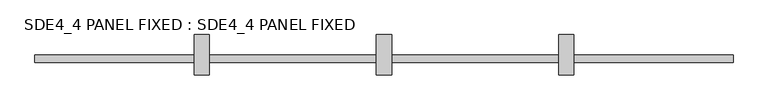
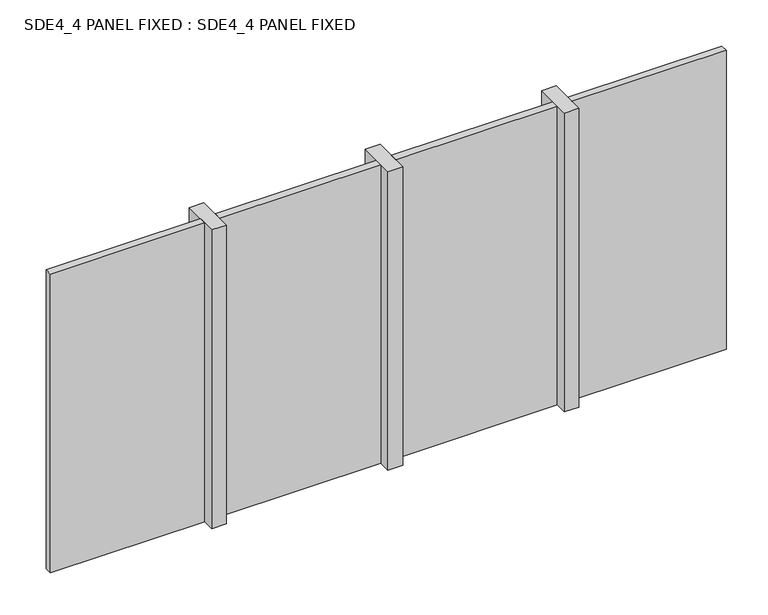
"""IFC4 building model written with IfcOpenShell, lengths in millimetres: plate geometry, SDE4_4 PANEL FIXED : SDE4_4 PANEL FIXED."""

from ifc_helpers import new_model, si_unit, origin, origin_with_axes, place, context, project, spatial, polyline, outline, extrude, source, transform, mapped, element, save


def sde4_4_panel_fixed_sde4_4_panel_fixed_497a13d3(model_context):
    return source(origin(), model_context, "Body", "SweptSolid", [
        extrude(outline(polyline([(-1150.0, -132.5), (-1250.0, -132.5), (-1250.0, 132.5), (-1150.0, 132.5), (-1150.0, -132.5)])), origin_with_axes(), (0.0, 0.0, 1.0), 2150.0),
        extrude(outline(polyline([(50.0, -132.5), (-50.0, -132.5), (-50.0, 132.5), (50.0, 132.5), (50.0, -132.5)])), origin_with_axes(), (0.0, 0.0, 1.0), 2150.0),
        extrude(outline(polyline([(1250.0, -132.5), (1150.0, -132.5), (1150.0, 132.5), (1250.0, 132.5), (1250.0, -132.5)])), origin_with_axes(), (0.0, 0.0, 1.0), 2150.0),
        extrude(outline(polyline([(2299.0, -50.0), (1250.0, -50.0), (1250.0, 0.0), (2299.0, 0.0), (2299.0, -50.0)])), origin_with_axes(), (0.0, 0.0, 1.0), 2150.0),
        extrude(outline(polyline([(1150.0, -50.0), (50.0, -50.0), (50.0, 0.0), (1150.0, 0.0), (1150.0, -50.0)])), origin_with_axes(), (0.0, 0.0, 1.0), 2150.0),
        extrude(outline(polyline([(-50.0, -50.0), (-1150.0, -50.0), (-1150.0, 0.0), (-50.0, 0.0), (-50.0, -50.0)])), origin_with_axes(), (0.0, 0.0, 1.0), 2150.0),
        extrude(outline(polyline([(-1250.0, -50.0), (-2300.0, -50.0), (-2300.0, 0.0), (-1250.0, 0.0), (-1250.0, -50.0)])), origin_with_axes(), (0.0, 0.0, 1.0), 2150.0),
    ])


if __name__ == "__main__":
    model = new_model("IFC4")
    model_context = context("Model", 3, world=origin())
    ifc_project = project(units=[si_unit("LENGTHUNIT", "METRE", prefix="MILLI")], contexts=[model_context])
    site = spatial("IfcSite", under=ifc_project)
    building = spatial("IfcBuilding", under=site)
    placement = place(None, origin())
    sde4_4_panel_fixed_sde4_4_panel_fixed_shape = sde4_4_panel_fixed_sde4_4_panel_fixed_497a13d3(model_context)
    element("IfcPlate", 1, ObjectType="SDE4_4 PANEL FIXED : SDE4_4 PANEL FIXED", at=placement, inside=building, context=model_context, shape_type="MappedRepresentation", body=[
        mapped(sde4_4_panel_fixed_sde4_4_panel_fixed_shape, transform((0.0, 0.0, 0.0), x_axis=(1.0, 0.0, 0.0), y_axis=(0.0, 1.0, 0.0), z_axis=(0.0, 0.0, 1.0))),
    ])
    save(model, "model.ifc")

# Revit data of these elements
# Type "SDE4_4 PANEL FIXED : SDE4_4 PANEL FIXED"
#   Type Mark = "CW-GLASS"
#   Analytic Construction = "<None>"
#   Glass = Glass
#   Frame = Aluminium
# Element 1 (IfcPlate, "SDE4_4 PANEL FIXED : SDE4_4 PANEL FIXED")
#   Materials on its faces: "Glass", "Aluminium"
# Materials
#   "Glass": class "Glass", colour RGB 0 128 192, transparency 0.9, Keynote = "L40", Cost = 0
#   "Aluminium": class "Unassigned", colour RGB 247 247 247, transparency 0, Cost = 0
